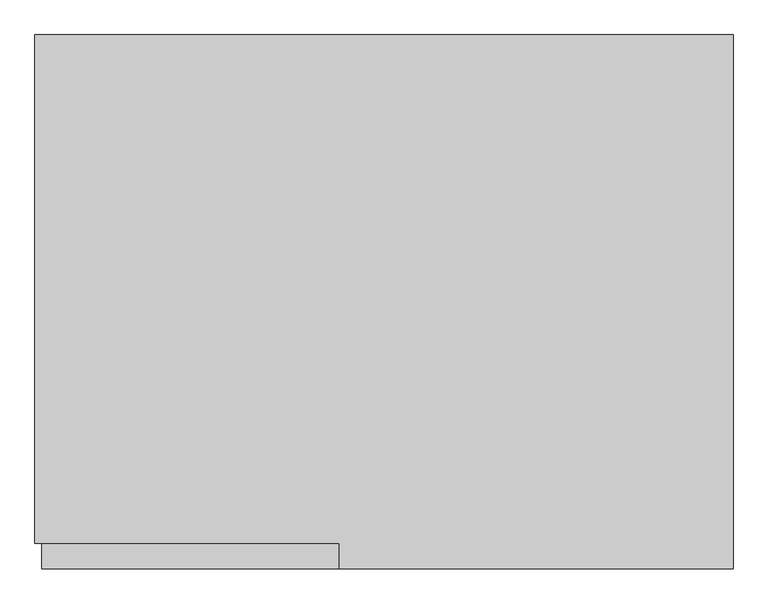
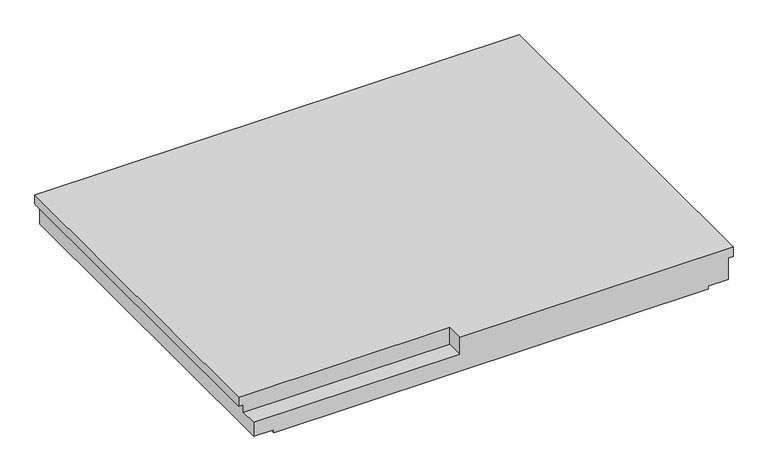
"""IFC4 building model written with IfcOpenShell, lengths in millimetres: proxy geometry, NLRS_24_GM_UN_rechthoekig bordes prefab zonder oplegnok-AV_gen_rsf : prefab bordes_gen__2300x3005."""

from ifc_helpers import new_model, si_unit, origin, place, context, project, spatial, faceted_brep, source, transform, mapped, element, save


def generic_models_1f0cb1f1(model_context):
    return source(origin(), model_context, "Body", "Brep", [
        faceted_brep([(1502.5, -2300.0, 0.0), (1502.5, -2300.0, -60.0), (1502.5, 0.0, -60.0), (1502.5, 0.0, 0.0), (-192.5, -2300.0, 0.0), (-192.5, -2190.0, 0.0), (-192.5, -2190.0, -110.0), (-192.5, -2300.0, -110.0), (-1502.5, 0.0, 0.0), (-1502.5, 0.0, -60.0), (-1502.5, -2190.0, -60.0), (-1502.5, -2190.0, 0.0), (-1472.5, -2300.0, -110.0), (-1472.5, -2300.0, -200.0), (-1347.5, -2300.0, -200.0), (-1347.5, -2300.0, -220.0), (1347.5, -2300.0, -220.0), (1347.5, -2300.0, -200.0), (1472.5, -2300.0, -200.0), (1472.5, -2300.0, -60.0), (-1472.5, -2190.0, -110.0), (-1472.5, -2190.0, -60.0), (1472.5, 0.0, -60.0), (1472.5, 0.0, -200.0), (1347.5, 0.0, -200.0), (1347.5, 0.0, -220.0), (-1347.5, 0.0, -220.0), (-1347.5, 0.0, -200.0), (-1472.5, 0.0, -200.0), (-1472.5, 0.0, -60.0)], [[[0, 1, 2, 3]], [[4, 5, 6, 7]], [[8, 9, 10, 11]], [[12, 13, 14, 15, 16, 17, 18, 19, 1, 0, 4, 7]], [[7, 6, 20, 12]], [[11, 10, 21, 20, 6, 5]], [[11, 5, 4, 0, 3, 8]], [[8, 3, 2, 22, 23, 24, 25, 26, 27, 28, 29, 9]], [[26, 25, 16, 15]], [[21, 10, 9, 29]], [[13, 12, 20, 21, 29, 28]], [[28, 27, 14, 13]], [[27, 26, 15, 14]], [[22, 2, 1, 19]], [[19, 18, 23, 22]], [[18, 17, 24, 23]], [[17, 16, 25, 24]]]),
    ])


if __name__ == "__main__":
    model = new_model("IFC4")
    model_context = context("Model", 3, world=origin())
    ifc_project = project(units=[si_unit("LENGTHUNIT", "METRE", prefix="MILLI")], contexts=[model_context])
    site = spatial("IfcSite", under=ifc_project)
    building = spatial("IfcBuilding", under=site)
    placement = place(None, origin())
    generic_models_shape = generic_models_1f0cb1f1(model_context)
    element("IfcBuildingElementProxy", 1, Name="NLRS_24_GM_UN_rechthoekig bordes prefab zonder oplegnok-AV_gen_rsf : prefab bordes_gen__2300x3005", ObjectType="NLRS_24_GM_UN_rechthoekig bordes prefab zonder oplegnok-AV_gen_rsf : prefab bordes_gen__2300x3005", at=placement, inside=building, context=model_context, shape_type="MappedRepresentation", body=[
        mapped(generic_models_shape, transform((0.0, 0.0, 0.0), x_axis=(1.0, 0.0, 0.0), y_axis=(0.0, 1.0, 0.0), z_axis=(0.0, 0.0, 1.0))),
    ])
    save(model, "model.ifc")

# Revit data of these elements
# Type "NLRS_24_GM_UN_rechthoekig bordes prefab zonder oplegnok-AV_gen_rsf : prefab bordes_gen__2300x3005"
#   Export Type to IFC As = "IfcStair"
#   Type IfcGUID = "2CEqVLPNH8KRN7ghwV3agL"
#   Type Comments = " "
#   Model = " "
#   Manufacturer = " "
#   Description = "rechthoekig bordes prefab\r\n1930x4395"
#   Assembly Code = "24.15"
#   Width = 3005 mm
#   Thickness = 220 mm
#   Perimeter = 10610 mm
#   NLRS_C_lengte_02 = 1310 mm
#   NLRS_C_lengte_01 = 1310 mm
#   NLRS_C_hoogte_02 = 110 mm
#   NLRS_C_hoogte_01 = 110 mm
#   NLRS_C_diepte_04 = 2300 mm
#   NLRS_C_diepte_03 = 2300 mm
#   NLRS_C_diepte_02 = 110 mm
#   NLRS_C_diepte_01 = 110 mm
#   Length = 2300 mm
#   Default Elevation = 1219.2 mm
#   Area = 6.9115 m²
#   NLRS_C_materiaal = NLRS_f2_beton prefab_gen_rsf
#   Keynote = ""
# Element 1 (IfcBuildingElementProxy, "NLRS_24_GM_UN_rechthoekig bordes prefab zonder oplegnok-AV_gen_rsf : prefab bordes_gen__2300x3005")
#   Materials on its faces: "NLRS_f2_beton prefab_gen_rsf"
# Materials
#   "NLRS_f2_beton prefab_gen_rsf": class "F - Niet gebakken kunststeen", colour RGB 129 133 118, transparency 0, Keynote = "f2", Manufacturer = "Revit Standards Foundation", URL = "www.revitstandards.org", Description = "beton prefab", Cost = 0
